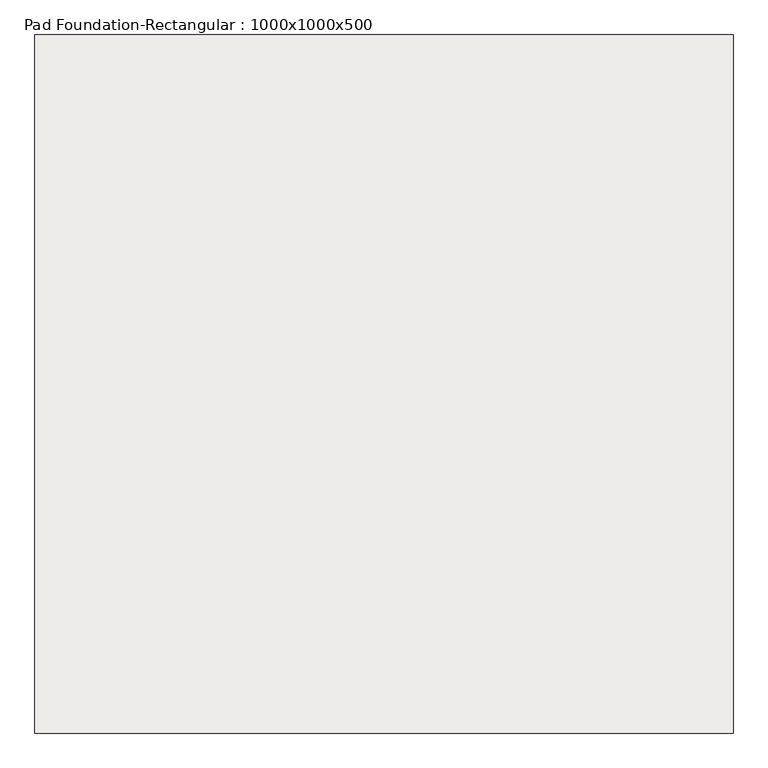
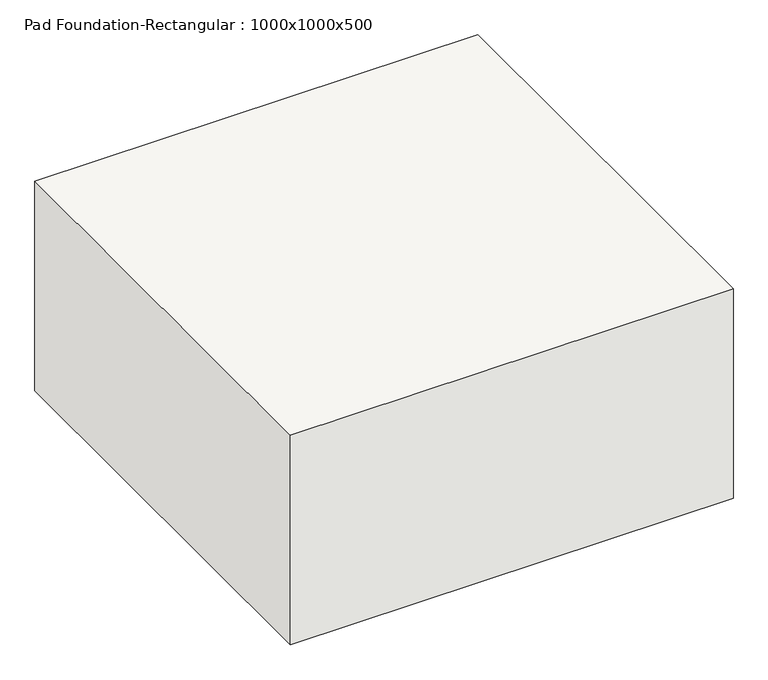
"""IFC4 building model written with IfcOpenShell, lengths in millimetres: slab geometry, Pad Foundation-Rectangular : 1000x1000x500."""

import ifcopenshell
import ifcopenshell.guid

model = None  # the IFC model being written
_history = None  # IfcOwnerHistory: only IFC2X3 demands one
_inside = {}  # id of a spatial element -> (the spatial element, [elements in it])
_under = {}  # id of a project, library or spatial element -> (it, [spatial elements below it])
_declared = {}  # id of a project -> (the project, [libraries it declares])
_typed = {}  # id of a type object -> (the type object, [elements of that type])
_made_of = {}  # id of a material, layer set ... -> (it, [elements and type objects made of it])


def new_model(schema):
    """Start an empty IFC model of exactly this schema.

    Asked for "IFC4X3", IfcOpenShell would pick the latest addendum, in which some entities
    have other attributes; the version numbers below select the first issue.
    IFC2X3 requires an IfcOwnerHistory on every rooted entity: one is made here for all.
    """
    global model, _history
    if schema == "IFC4X3":
        model = ifcopenshell.file(schema_version=(4, 3, 0, 0))
    else:
        model = ifcopenshell.file(schema=schema)
    _inside.clear()
    _under.clear()
    _declared.clear()
    _typed.clear()
    _made_of.clear()
    _history = None
    if model.schema == "IFC2X3":
        org = make("IfcOrganization", Name="unknown")
        user = make(
            "IfcPersonAndOrganization",
            ThePerson=make("IfcPerson", FamilyName="unknown"),
            TheOrganization=org,
        )
        app = make(
            "IfcApplication",
            ApplicationDeveloper=org,
            Version="unknown",
            ApplicationFullName="unknown",
            ApplicationIdentifier="unknown",
        )
        _history = make(
            "IfcOwnerHistory",
            OwningUser=user,
            OwningApplication=app,
            ChangeAction="ADDED",
            CreationDate=0,
        )
    return model


def make(cls, **values):
    """One entity of the class cls with the attributes given. An attribute that is None is left unset."""
    return model.create_entity(
        cls, **{name: value for name, value in values.items() if value is not None}
    )


def rooted(cls, **values):
    """An entity with a GlobalId (a new one), such as an element, a storey or a relation."""
    return make(cls, GlobalId=ifcopenshell.guid.new(), OwnerHistory=_history, **values)


def si_unit(unit_type, name, prefix=None):
    """IfcSIUnit, for example si_unit("LENGTHUNIT", "METRE", prefix="MILLI")."""
    return make("IfcSIUnit", UnitType=unit_type, Prefix=prefix, Name=name)


def assignment(units):
    """IfcUnitAssignment: the units of a project."""
    return None if units is None else make("IfcUnitAssignment", Units=units)


def point(xyz):
    """IfcCartesianPoint."""
    return None if xyz is None else make("IfcCartesianPoint", Coordinates=xyz)


def direction(xyz):
    """IfcDirection."""
    return None if xyz is None else make("IfcDirection", DirectionRatios=xyz)


def frame(location, z_axis=None, x_axis=None):
    """IfcAxis2Placement3D, a coordinate frame: its origin and axes. An axis left out is left unset."""
    return make(
        "IfcAxis2Placement3D",
        Location=point(location),
        Axis=direction(z_axis),
        RefDirection=direction(x_axis),
    )


def origin():
    """The frame at (0, 0, 0) with its axes left unset."""
    return frame((0.0, 0.0, 0.0))


def place(relative_to, where):
    """IfcLocalPlacement: puts the frame where relative to a parent placement (None: the world)."""
    return make(
        "IfcLocalPlacement", PlacementRelTo=relative_to, RelativePlacement=where
    )


def context(
    kind, dimensions, precision=None, world=None, true_north=None, identifier=None
):
    """IfcGeometricRepresentationContext, for example the 3D "Model" context."""
    return make(
        "IfcGeometricRepresentationContext",
        ContextIdentifier=identifier,
        ContextType=kind,
        CoordinateSpaceDimension=dimensions,
        Precision=precision,
        WorldCoordinateSystem=world,
        TrueNorth=true_north,
    )


def project(units=None, contexts=None):
    """IfcProject with its units and contexts."""
    return rooted(
        "IfcProject",
        Name="project",
        RepresentationContexts=contexts,
        UnitsInContext=assignment(units),
    )


def spatial(cls, under=None, at=None, **own):
    """A site, building, storey or space (cls), placed at a placement, below another one or the project."""
    s = rooted(cls, ObjectPlacement=at, **own)
    if under is not None:
        _under.setdefault(under.id(), (under, []))[1].append(s)
    return s


def polyline(points):
    """IfcPolyline through the points."""
    return make("IfcPolyline", Points=[point(p) for p in points])


def outline(outer, holes=None, kind="AREA"):
    """IfcArbitraryClosedProfileDef: a profile drawn as a closed curve; with holes, ...WithVoids."""
    if holes is None:
        return make("IfcArbitraryClosedProfileDef", ProfileType=kind, OuterCurve=outer)
    return make(
        "IfcArbitraryProfileDefWithVoids",
        ProfileType=kind,
        OuterCurve=outer,
        InnerCurves=holes,
    )


def extrude(swept, where, along, depth):
    """IfcExtrudedAreaSolid: the profile swept, set in the frame where, extruded along a direction by depth."""
    return make(
        "IfcExtrudedAreaSolid",
        SweptArea=swept,
        Position=where,
        ExtrudedDirection=direction(along),
        Depth=depth,
    )


def shape(context_of_items, identifier, shape_type, items):
    """IfcShapeRepresentation: the items that make up one representation, for example the "Body"."""
    return make(
        "IfcShapeRepresentation",
        ContextOfItems=context_of_items,
        RepresentationIdentifier=identifier,
        RepresentationType=shape_type,
        Items=items,
    )


def source(mapping_origin, context_of_items, identifier, shape_type, items):
    """IfcRepresentationMap: a shape defined once, which mapped items show again and again."""
    return make(
        "IfcRepresentationMap",
        MappingOrigin=mapping_origin,
        MappedRepresentation=shape(context_of_items, identifier, shape_type, items),
    )


def transform(
    local_origin,
    x_axis=None,
    y_axis=None,
    z_axis=None,
    scale=None,
    scale2=None,
    scale3=None,
    uniform=True,
):
    """IfcCartesianTransformationOperator3D, or its non-uniform kind. x_axis, y_axis, z_axis: its Axis1, 2, 3."""
    if uniform:
        return make(
            "IfcCartesianTransformationOperator3D",
            Axis1=direction(x_axis),
            Axis2=direction(y_axis),
            LocalOrigin=point(local_origin),
            Scale=scale,
            Axis3=direction(z_axis),
        )
    return make(
        "IfcCartesianTransformationOperator3DnonUniform",
        Axis1=direction(x_axis),
        Axis2=direction(y_axis),
        LocalOrigin=point(local_origin),
        Scale=scale,
        Axis3=direction(z_axis),
        Scale2=scale2,
        Scale3=scale3,
    )


def mapped(mapping_source, mapping_target):
    """IfcMappedItem: shows the shape of a source again, moved by a transform."""
    return make(
        "IfcMappedItem", MappingSource=mapping_source, MappingTarget=mapping_target
    )


def made_of(thing, what):
    """Note that an element or type object is made of a material, layer set ...; save() writes the relation."""
    if what is not None:
        _made_of.setdefault(what.id(), (what, []))[1].append(thing)
    return thing


def element(
    cls,
    number,
    at=None,
    inside=None,
    cuts=None,
    type_object=None,
    material=None,
    context=None,
    identifier="Body",
    shape_type=None,
    held_by="IfcProductDefinitionShape",
    body=None,
    shapes=None,
    **own,
):
    """One element of the class cls, such as IfcWall. Its Tag is "e" and its number.

    at: its placement. inside: the storey or other place that contains it. cuts: it is an
    opening in that element (IfcRelVoidsElement). A single representation is given by context,
    identifier, shape_type and body (its items); several are given by shapes. held_by: the class
    of the entity that holds the representations. save() writes the other relations.
    """
    e = rooted(cls, Tag="e%d" % number, ObjectPlacement=at, **own)
    if body is not None:
        shapes = [shape(context, identifier, shape_type, body)]
    if shapes is not None:
        e.Representation = make(held_by, Representations=shapes)
    if inside is not None:
        _inside.setdefault(inside.id(), (inside, []))[1].append(e)
    if cuts is not None:
        rooted(
            "IfcRelVoidsElement", RelatingBuildingElement=cuts, RelatedOpeningElement=e
        )
    if type_object is not None:
        _typed.setdefault(type_object.id(), (type_object, []))[1].append(e)
    return made_of(e, material)


def aggregate(whole, parts):
    """IfcRelAggregates: a whole, such as a stair, and the parts it consists of."""
    return rooted("IfcRelAggregates", RelatingObject=whole, RelatedObjects=parts)


def save(model, path):
    """Write the relations noted so far, then the file.

    IfcRelAggregates (storeys below a building ...), IfcRelContainedInSpatialStructure (elements
    in a storey), IfcRelDefinesByType, IfcRelAssociatesMaterial and IfcRelDeclares: one each for
    every whole, place, type object, material and project.
    """
    for whole, parts in _under.values():
        aggregate(whole, parts)
    for where, things in _inside.values():
        rooted(
            "IfcRelContainedInSpatialStructure",
            RelatedElements=things,
            RelatingStructure=where,
        )
    for kind, things in _typed.values():
        rooted("IfcRelDefinesByType", RelatedObjects=things, RelatingType=kind)
    for what, things in _made_of.values():
        rooted("IfcRelAssociatesMaterial", RelatedObjects=things, RelatingMaterial=what)
    for by, libraries in _declared.values():
        rooted("IfcRelDeclares", RelatingContext=by, RelatedDefinitions=libraries)
    model.write(path)


def pad_foundation_rectangular_1000x1000x500_ed6229e9(model_context):
    return source(origin(), model_context, "Body", "SweptSolid", [
        extrude(outline(polyline([(500.0, 500.0), (500.0, -500.0), (-500.0, -500.0), (-500.0, 500.0), (500.0, 500.0)])), frame((0.0, 0.0, -500.0), z_axis=(0.0, 0.0, 1.0), x_axis=(1.0, 0.0, 0.0)), (0.0, 0.0, 1.0), 500.0),
    ])


if __name__ == "__main__":
    model = new_model("IFC4")
    model_context = context("Model", 3, world=origin())
    ifc_project = project(units=[si_unit("LENGTHUNIT", "METRE", prefix="MILLI")], contexts=[model_context])
    site = spatial("IfcSite", under=ifc_project)
    building = spatial("IfcBuilding", under=site)
    placement = place(None, origin())
    pad_foundation_rectangular_1000x1000x500_shape = pad_foundation_rectangular_1000x1000x500_ed6229e9(model_context)
    element("IfcSlab", 1, ObjectType="Pad Foundation-Rectangular : 1000x1000x500", at=placement, inside=building, context=model_context, shape_type="MappedRepresentation", body=[
        mapped(pad_foundation_rectangular_1000x1000x500_shape, transform((0.0, 0.0, 0.0), x_axis=(1.0, 0.0, 0.0), y_axis=(0.0, 1.0, 0.0), z_axis=(0.0, 0.0, 1.0))),
    ])
    save(model, "model.ifc")

# Revit data of these elements
# Project information
#   Project Status = "Project Status"
#   Client Name = "Revit Project"
#   Project Address = "LIMERICK INSTITUTE of TECHNOLOGY"
#   Project Name = "Commercial Units"
#   Project Number = "01"
# Type "Pad Foundation-Rectangular : 1000x1000x500"
#   Reinforcement Specs [instance default] = ""
#   Pad Type = "P1"
#   Mesh [instance default] = ""
#   Concrete Grade [instance default] = ""
#   Volume = 0.50 m³
#   Pad Width = 1000 mm
#   Pad Length = 1000 mm
#   Pad Depth = 500 mm
#   Structural Material [instance default] = Concrete - Cast-in-Place Concrete
# Element 1 (IfcSlab, "Pad Foundation-Rectangular : 1000x1000x500")
#   Materials on its faces: "Concrete - Cast-in-Place Concrete"
# Materials
#   "Concrete - Cast-in-Place Concrete": class "Concrete", colour RGB 192 192 192, transparency 0
